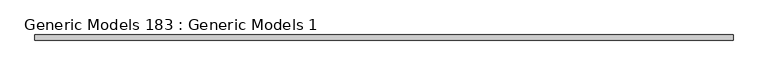
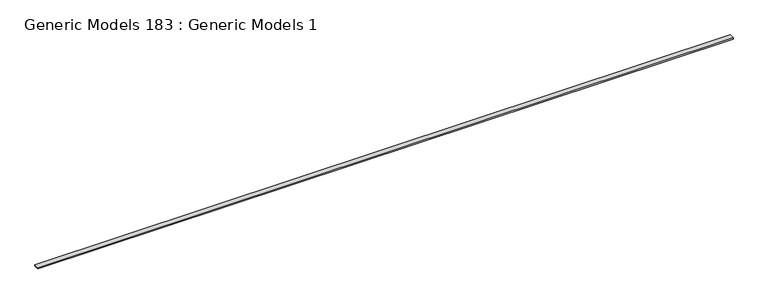
"""IFC4 building model written with IfcOpenShell, lengths in millimetres: proxy geometry, Generic Models 183 : Generic Models 1."""

from ifc_helpers import new_model, si_unit, frame, origin, place, context, project, spatial, polyline, outline, extrude, source, transform, mapped, element, save


def generic_models_183_generic_models_1_4846466b(model_context):
    return source(origin(), model_context, "Body", "SweptSolid", [
        extrude(outline(polyline([(-10459.9421316, -7106.2230338), (-10459.9421316, -6966.5230338), (8590.0578684, -6966.5230338), (8590.0578684, -7106.2230338), (-10459.9421316, -7106.2230338)])), frame((0.0, 0.0, 126955.296), z_axis=(0.0, 0.0, 1.0), x_axis=(1.0, 0.0, 0.0)), (0.0, 0.0, 1.0), 38.1),
    ])


if __name__ == "__main__":
    model = new_model("IFC4")
    model_context = context("Model", 3, world=origin())
    ifc_project = project(units=[si_unit("LENGTHUNIT", "METRE", prefix="MILLI")], contexts=[model_context])
    site = spatial("IfcSite", under=ifc_project)
    building = spatial("IfcBuilding", under=site)
    placement = place(None, origin())
    generic_models_183_generic_models_1_shape = generic_models_183_generic_models_1_4846466b(model_context)
    element("IfcBuildingElementProxy", 1, Name="Generic Models 183 : Generic Models 1", ObjectType="Generic Models 183 : Generic Models 1", at=placement, inside=building, context=model_context, shape_type="MappedRepresentation", body=[
        mapped(generic_models_183_generic_models_1_shape, transform((0.0, 0.0, 0.0), x_axis=(1.0, 0.0, 0.0), y_axis=(0.0, 1.0, 0.0), z_axis=(0.0, 0.0, 1.0))),
    ])
    save(model, "model.ifc")

# Revit data of these elements
# Element 1 (IfcBuildingElementProxy, "Generic Models 183 : Generic Models 1")
#   Materials on its faces: "_2X BLOCKING AS REQUIRED"
# Materials
#   "_2X BLOCKING AS REQUIRED": class "Generic", colour RGB 177 130 114, transparency 0, Cost = 0
